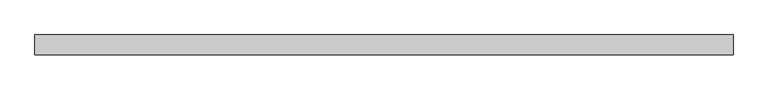
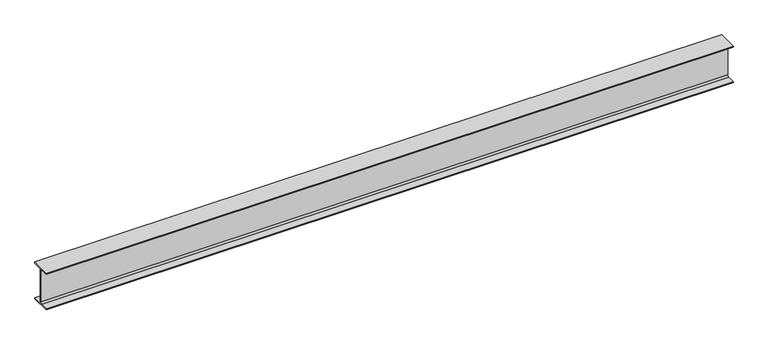
"""IFC4 building model written with IfcOpenShell, lengths in millimetres: beam geometry, 0912_Steel Framing_H-KSD3502 : H_SB_ASB_H-350x175x7x11."""

from ifc_helpers import new_model, si_unit, point, frame, frame_2d, origin, place, context, project, spatial, polyline, circle_curve, trimmed, segment, composite_curve, outline, extrude, source, transform, mapped, element, save


def beam_a4f2fb3b(model_context):
    return source(origin(), model_context, "Body", "SweptSolid", [
        extrude(outline(composite_curve([segment(polyline([(87.5, -164.0), (87.5, -175.0), (-87.5, -175.0), (-87.5, -164.0), (-17.5, -164.0)]), True, "CONTINUOUS"), segment(trimmed(circle_curve(frame_2d((-17.5, -150.0)), 14.0), [point((-17.5, -164.0))], [point((-3.5, -150.0))], True, "CARTESIAN"), True, "CONTINUOUS"), segment(polyline([(-3.5, -150.0), (-3.5, 150.0)]), True, "CONTINUOUS"), segment(trimmed(circle_curve(frame_2d((-17.5, 150.0)), 14.0), [point((-3.5, 150.0))], [point((-17.5, 164.0))], True, "CARTESIAN"), True, "CONTINUOUS"), segment(polyline([(-17.5, 164.0), (-87.5, 164.0), (-87.5, 175.0), (87.5, 175.0), (87.5, 164.0), (17.5, 164.0)]), True, "CONTINUOUS"), segment(trimmed(circle_curve(frame_2d((17.5, 150.0)), 14.0), [point((17.5, 164.0))], [point((3.5, 150.0))], True, "CARTESIAN"), True, "CONTINUOUS"), segment(polyline([(3.5, 150.0), (3.5, -150.0)]), True, "CONTINUOUS"), segment(trimmed(circle_curve(frame_2d((17.5, -150.0)), 14.0), [point((3.5, -150.0))], [point((17.5, -164.0))], True, "CARTESIAN"), True, "CONTINUOUS"), segment(polyline([(17.5, -164.0), (87.5, -164.0)]), True, "CONTINUOUS")], self_intersect=False)), frame((-3087.3, 0.0, 0.0), z_axis=(1.0, 0.0, 0.0), x_axis=(0.0, 1.0, 0.0)), (0.0, 0.0, 1.0), 6174.6),
    ])


if __name__ == "__main__":
    model = new_model("IFC4")
    model_context = context("Model", 3, world=origin())
    ifc_project = project(units=[si_unit("LENGTHUNIT", "METRE", prefix="MILLI")], contexts=[model_context])
    site = spatial("IfcSite", under=ifc_project)
    building = spatial("IfcBuilding", under=site)
    placement = place(None, origin())
    beam_shape = beam_a4f2fb3b(model_context)
    element("IfcBeam", 1, ObjectType="0912_Steel Framing_H-KSD3502 : H_SB_ASB_H-350x175x7x11", at=placement, inside=building, context=model_context, shape_type="MappedRepresentation", body=[
        mapped(beam_shape, transform((0.0, 0.0, 0.0), x_axis=(1.0, 0.0, 0.0), y_axis=(0.0, 1.0, 0.0), z_axis=(0.0, 0.0, 1.0))),
    ])
    save(model, "model.ifc")

# Revit data of these elements
# Type "0912_Steel Framing_H-KSD3502 : H_SB_ASB_H-350x175x7x11"
#   H_WM Code_1 = "S01AA002-00001 | Main Steel Structure Fabrication Work | Shelter/Building | Medium Steel - Standard (90KG/M>Weight≥30KG/M) | Material: (   )"
#   H_WM Code_2 = "S03AA028-00001 | Main Steel Structure Erection Work | Shelter/Building | Medium Steel (90KG/M>Weight≥30KG/M) | Material: (   )"
#   H_WM Code_3 = "S01AA010-00001 | Main Steel Structure Fabrication Work | Shelter/Building | Steel Painting/Coating | for Non-Fireproofed Steel Surface, Surface Preparation, Primer, Second & Final Coat | Material: (   )"
#   H_Q'ty Cal Type Tag = "SB-Q2"
#   Width = 17.5 cm
#   Web Thickness = 0.7 cm
#   Web Fillet = 1.4 cm
#   Warping Constant = 282000.0 cm⁶
#   W = 0
#   Torsional Moment of Inertia = 19.4042 cm⁴
#   Section Area = 63.14 cm²
#   Plastic Modulus weak axis = 174.0 cm³
#   Plastic Modulus strong axis = 868.0 cm³
#   Perimeter = 1.36 m²/m
#   Nominal Weight = 49.60 kgf/m
#   Moment of Inertia weak axis = 984.00 cm⁴
#   Moment of Inertia strong axis = 13600.00 cm⁴
#   Height = 35.0 cm
#   Flange Thickness = 1.1 cm
#   Elastic Modulus weak axis = 112.0 cm³
#   Elastic Modulus strong axis = 775.0 cm³
#   Centroid Vertical = 17.5 cm
#   Centroid Horizontal = 8.75 cm
#   Ix = 136000000
#   Length [instance default] = 1.5240 m
#   Zx = 868000
#   b = 0.1750 m
#   h = 0.3500 m
#   r = 0.0140 m
#   s = 0.0070 m
#   t = 0.0110 m
#   A = 0.006314 m²
#   Structural Material [instance default] = Steel, 45-345
#   Assembly Code = ""
# Element 1 (IfcBeam, "0912_Steel Framing_H-KSD3502 : H_SB_ASB_H-350x175x7x11")
#   Structural Material = none
# Materials
#   "Steel, 45-345": class "Metal", colour RGB 189 187 185, transparency 0, Description = "Steel 345 MPa", Cost = 0
